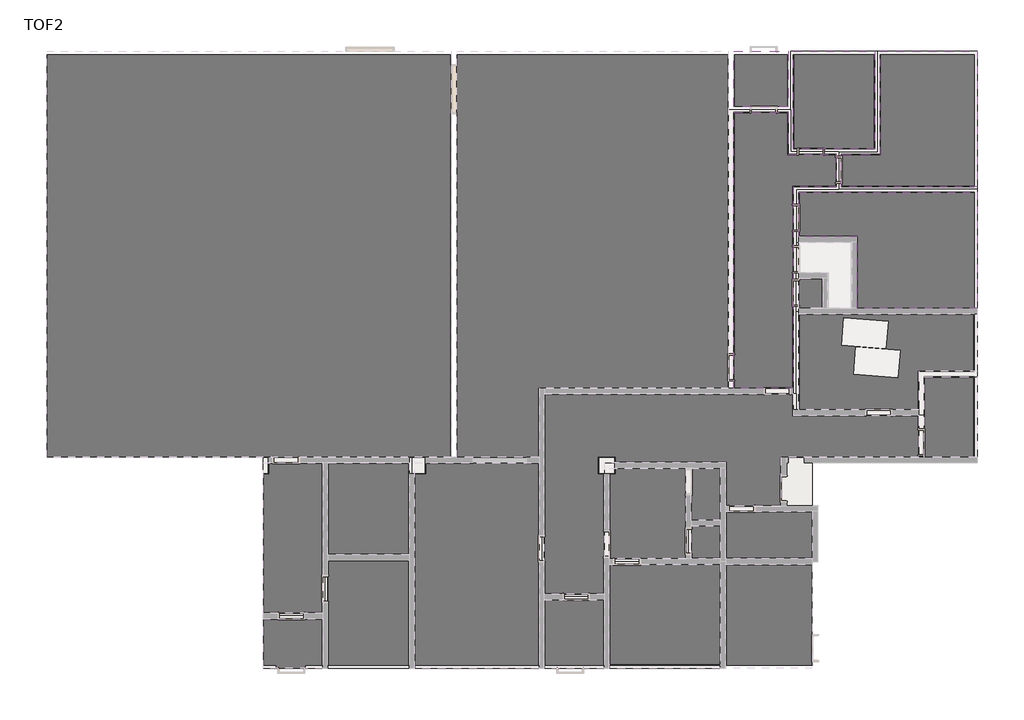
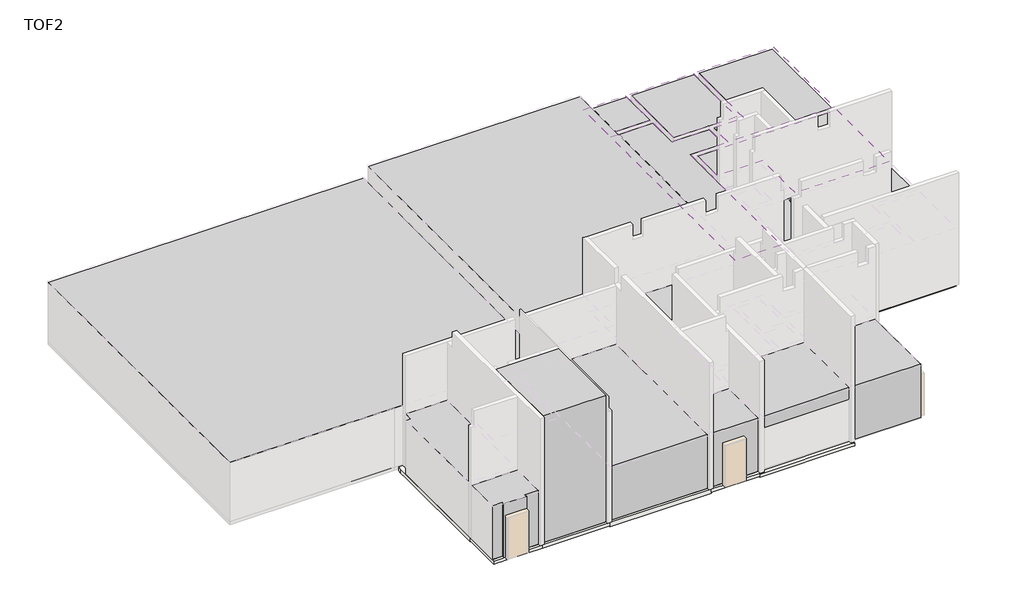
# One storey, part 5 of 5: 24 slabs, 23 proxies, 5 coverings.
# Revit data of these elements (continued)
# Room at (9390, 17931.521) mm, phase "New Construction", upper level "TOC", upper offset 2000 mm, lower offset -1000 mm (continued)
#   H_Ceiling-Base Material-5 = ""
#   H_Ceiling Finish-1 = "Acrylic Emulsion Paint"
#   H_Ceiling Finish-2 = ""
#   H_Ceiling Finish Remark = "SACE"
#   H_Room W = 17700 mm
#   H_Room L = 11400 mm
#   H_Room H or CH = 7300 mm
#   Floor Finish Style No = F06A
#   Skirt Finish Style No = B03
#   Wall Finish Style No = W01B
#   Ceiling Finish Style No = C01
# Room at (9390, 6347.521) mm, phase "New Construction", upper level "TOC", upper offset 2000 mm, lower offset -1000 mm
#   Comments = ""
#   Number = "112"
#   Name = "ELECTRICAL ROOM(SS08)"
#   H_Floor Finish Style Name = "Non-Slip Epoxy Paint"
#   H_Floor Base Material = "Concrete Slab / Screed"
#   H_Wall-Base Material-1 = "Masonry Wall"
#   H_Skirt Finish Style Name = "Epoxy Paint"
#   H_Wall-Base Material-2 = ""
#   H_Wall-Base Material-3 = "Plastering"
#   H_Floor-Base Material-1 = "Concrete Slab"
#   H_Floor-Base Material-2 = ""
#   H_Floor-Base Material-3 = "Screed"
#   H_Floor-Base Material-4 = ""
#   H_Floor-Base Material-5 = ""
#   H_Floor Finish-1 = "Epoxy Paint"
#   H_Floor Finish-2 = ""
#   H_Floor Finish Remark = "*WM 기준 확인 필요 Epoxy Paint \n(용제형, 0.1mm 이하) : epoxy resin + polyamine hardener(경화제)"
#   H_Skirt Base Material = "Same as Wall"
#   H_Skirt-Base Material-1 = ""
#   H_Skirt-Base Material-2 = ""
#   H_Skirt-Base Material-3 = ""
#   H_Skirt-Base Material-4 = ""
#   H_Skirt-Base Material-5 = ""
#   H_Skirt Finish-1 = "Epoxy Paint"
#   H_Skirt Finish-2 = ""
#   H_Skirt Finish Remark = "SACE"
#   H_Wall Finish Style Name = "Acrylic Emulsion Paint"
#   H_Wall Base Material = "Masonry Wall / Cement Plaster"
#   H_Wall-Base Material-4 = ""
#   H_Wall-Base Material-5 = ""
#   H_Wall Finish-1 = "Acrylic Emulsion Paint"
#   H_Wall Finish-2 = ""
#   H_Wall Finish Remark = "T13 Plaster"
#   H_Ceiling Finish Style Name = "Acrylic Emulsion Paint"
#   H_Ceiling Base Material = "Concrete Slab / Fair Faced Concrete"
#   H_Ceiling-Base Material-1 = "(Concrete Slab)"
#   H_Ceiling-Base Material-2 = ""
#   H_Ceiling-Base Material-3 = ""
#   H_Ceiling-Base Material-4 = ""
#   H_Ceiling-Base Material-5 = ""
#   H_Ceiling Finish-1 = "Acrylic Emulsion Paint"
#   H_Ceiling Finish-2 = ""
#   H_Ceiling Finish Remark = "SACE"
#   H_Room W = 17700 mm
#   H_Room L = 11000 mm
#   H_Room H or CH = 7300 mm
#   Floor Finish Style No = F06B
#   Skirt Finish Style No = B03
#   Wall Finish Style No = W01B
#   Ceiling Finish Style No = C01
# Room at (25850, 15981.521) mm, phase "New Construction", upper level "TOC", upper offset 2000 mm, lower offset 0 mm
#   Comments = ""
#   Number = "102"
#   Name = "RACK ROOM"
#   H_Floor Finish Style Name = "Anti-Dust Epoxy Paint / Anti-Static Vinyl Tile on Raised Floor"
#   H_Floor Base Material = "Concrete Slab / Steel Trowel Finish"
#   H_Wall-Base Material-1 = "Masonry Wall"
#   H_Skirt Finish Style Name = "Coved Vinyl Tile"
#   H_Wall-Base Material-2 = ""
#   H_Wall-Base Material-3 = "Plastering"
#   H_Floor-Base Material-1 = "Concrete Slab"
#   H_Floor-Base Material-2 = "Steel Trowel Finish"
#   H_Floor-Base Material-3 = ""
#   H_Floor-Base Material-4 = ""
#   H_Floor-Base Material-5 = "Raised Floor_Anti-Static Vinyl Tile"
#   H_Floor Finish-1 = "Anti-Dust Paint"
#   H_Floor Finish-2 = "Raised Floor_Anti-Static Vinyl Tile"
#   H_Floor Finish Remark = "600x600, H=1000"
#   H_Skirt Base Material = "Same as Wall"
#   H_Skirt-Base Material-1 = ""
#   H_Skirt-Base Material-2 = ""
#   H_Skirt-Base Material-3 = ""
#   H_Skirt-Base Material-4 = ""
#   H_Skirt-Base Material-5 = ""
#   H_Skirt Finish-1 = "Vinyl Tile"
#   H_Skirt Finish-2 = ""
#   H_Skirt Finish Remark = "Vinyl Tile = PVC Tile (polyvinyl chloride)"
#   H_Wall Finish Style Name = "Acrylic Emulsion Paint"
#   H_Wall Base Material = "Masonry Wall / Cement Plaster"
#   H_Wall-Base Material-4 = ""
#   H_Wall-Base Material-5 = ""
#   H_Wall Finish-1 = "Acrylic Emulsion Paint"
#   H_Wall Finish-2 = ""
#   H_Wall Finish Remark = "T13 Plaster"
#   H_Ceiling Finish Style Name = "Suspended Acoustic Tiled Ceiling (M-Bar)"
#   H_Ceiling Base Material = "Concrete Slab / Fair Faced Concrete"
#   H_Ceiling-Base Material-1 = "(Concrete Slab)"
#   H_Ceiling-Base Material-2 = "(Fair Faced Concrete)"
#   H_Ceiling-Base Material-3 = ""
#   H_Ceiling-Base Material-4 = ""
#   H_Ceiling-Base Material-5 = "Acoustic Tiled Ceiling System (M-Bar)"
#   H_Ceiling Finish-1 = "Acoustic Tiled Ceiling System (M-Bar)"
#   H_Ceiling Finish-2 = ""
#   H_Ceiling Finish Remark = ""
#   H_Room W = 14900 mm
#   H_Room L = 14900 mm
#   H_Room H or CH = 3000 mm
#   Floor Finish Style No = F91
#   Skirt Finish Style No = B35
#   Wall Finish Style No = W01B
#   Ceiling Finish Style No = C95A
# Room at (22100, 4784.521) mm, phase "New Construction", upper level "TOC", upper offset 2000 mm, lower offset -1000 mm
#   Comments = ""
#   Number = "114"
#   Name = "BATTERY ROOM"
#   H_Floor Finish Style Name = "Acid Resistant Ceramic Tile"
#   H_Floor Base Material = "Concrete Slab / Steel Trowel Finish"
#   H_Wall-Base Material-1 = "Masonry Wall"
#   H_Skirt Finish Style Name = "Coved Vinyl Tile"
#   H_Wall-Base Material-2 = ""
#   H_Wall-Base Material-3 = "Plastering"
#   H_Floor-Base Material-1 = "Concrete Slab"
#   H_Floor-Base Material-2 = "Steel Trowel Finish"
#   H_Floor-Base Material-3 = ""
#   H_Floor-Base Material-4 = ""
#   H_Floor-Base Material-5 = "Acid/Alkaline Resistant Tile"
#   H_Floor Finish-1 = "Acid/Alkaline Resistant Tile"
#   H_Floor Finish-2 = ""
#   H_Floor Finish Remark = "*WM : Bonding용 Mortar은 Tile에 포함\n*Slope 용 Screed만 별도 구분 (Concrete 바닥 단차 발생하는 경우 Only)"
#   H_Skirt Base Material = "Same as Wall"
#   H_Skirt-Base Material-1 = ""
#   H_Skirt-Base Material-2 = ""
#   H_Skirt-Base Material-3 = ""
#   H_Skirt-Base Material-4 = ""
#   H_Skirt-Base Material-5 = ""
#   H_Skirt Finish-1 = "Vinyl Tile"
#   H_Skirt Finish-2 = ""
#   H_Skirt Finish Remark = "Vinyl Tile = PVC Tile (polyvinyl chloride)"
#   H_Wall Finish Style Name = "Acid Resistant Paint"
#   H_Wall Base Material = "Masonry Wall / Cement Plaster"
#   H_Wall-Base Material-4 = ""
#   H_Wall-Base Material-5 = ""
#   H_Wall Finish-1 = "Acid/Alkaline Resistant Paint"
#   H_Wall Finish-2 = ""
#   H_Wall Finish Remark = "T13 Plaster"
#   H_Ceiling Finish Style Name = "Acrylic Emulsion Paint"
#   H_Ceiling Base Material = "Concrete Slab / Fair Faced Concrete"
#   H_Ceiling-Base Material-1 = "(Concrete Slab)"
#   H_Ceiling-Base Material-2 = ""
#   H_Ceiling-Base Material-3 = ""
#   H_Ceiling-Base Material-4 = ""
#   H_Ceiling-Base Material-5 = ""
#   H_Ceiling Finish-1 = "Acrylic Emulsion Paint"
#   H_Ceiling Finish-2 = ""
#   H_Ceiling Finish Remark = "SACE"
#   H_Room W = 7700 mm
#   H_Room L = 7500 mm
#   H_Room H or CH = 7300 mm
#   Floor Finish Style No = F32A
#   Skirt Finish Style No = B35
#   Wall Finish Style No = W04B
#   Ceiling Finish Style No = C01
# Room at (34305, 4784.521) mm, phase "New Construction", upper level "TOC", upper offset 2000 mm, lower offset 0 mm
#   Comments = ""
#   Number = "118"
#   Name = "DRIVERS LOUNGE"
#   H_Floor Finish Style Name = "Vinyl Tile"
#   H_Floor Base Material = "Concrete Slab / Steel Trowel Finish"
#   H_Wall-Base Material-1 = "Masonry Wall"
#   H_Skirt Finish Style Name = "Coved Vinyl Tile"
#   H_Wall-Base Material-2 = ""
#   H_Wall-Base Material-3 = "Plastering"
#   H_Floor-Base Material-1 = "Concrete Slab"
#   H_Floor-Base Material-2 = "Steel Trowel Finish"
#   H_Floor-Base Material-3 = ""
#   H_Floor-Base Material-4 = ""
#   H_Floor-Base Material-5 = "Vinyl Tile"
#   H_Floor Finish-1 = "Vinyl Tile"
#   H_Floor Finish-2 = ""
#   H_Floor Finish Remark = ""
#   H_Skirt Base Material = "Same as Wall"
#   H_Skirt-Base Material-1 = ""
#   H_Skirt-Base Material-2 = ""
#   H_Skirt-Base Material-3 = ""
#   H_Skirt-Base Material-4 = ""
#   H_Skirt-Base Material-5 = ""
#   H_Skirt Finish-1 = "Vinyl Tile"
#   H_Skirt Finish-2 = ""
#   H_Skirt Finish Remark = "Vinyl Tile = PVC Tile (polyvinyl chloride)"
#   H_Wall Finish Style Name = "Acrylic Emulsion Paint"
#   H_Wall Base Material = "Masonry Wall / Cement Plaster"
#   H_Wall-Base Material-4 = ""
#   H_Wall-Base Material-5 = ""
#   H_Wall Finish-1 = "Acrylic Emulsion Paint"
#   H_Wall Finish-2 = ""
#   H_Wall Finish Remark = "T13 Plaster"
#   H_Ceiling Finish Style Name = "Suspended Acoustic Tiled Ceiling (M-Bar)"
#   H_Ceiling Base Material = "Concrete Slab / Fair Faced Concrete"
#   H_Ceiling-Base Material-1 = "(Concrete Slab)"
#   H_Ceiling-Base Material-2 = "(Fair Faced Concrete)"
#   H_Ceiling-Base Material-3 = ""
#   H_Ceiling-Base Material-4 = ""
#   H_Ceiling-Base Material-5 = "Acoustic Tiled Ceiling System (M-Bar)"
#   H_Ceiling Finish-1 = "Acoustic Tiled Ceiling System (M-Bar)"
#   H_Ceiling Finish-2 = ""
#   H_Ceiling Finish Remark = ""
#   H_Room W = 4500 mm
#   H_Room L = 7500 mm
#   H_Room H or CH = 2600 mm
#   Floor Finish Style No = F34A
#   Skirt Finish Style No = B35
#   Wall Finish Style No = W01B
#   Ceiling Finish Style No = C95A
# Room at (38540.953, 16104.521) mm, phase "New Construction", upper level "TOC", upper offset 2000 mm, lower offset 0 mm
#   Comments = ""
#   Number = "103"
#   Name = "CONTROL ROOM"
#   H_Floor Finish Style Name = "Anti-Dust Epoxy Paint / Anti-Static Vinyl Tile on Raised Floor"
#   H_Floor Base Material = "Concrete Slab / Steel Trowel Finish"
#   H_Wall-Base Material-1 = "Masonry Wall"
#   H_Skirt Finish Style Name = "Coved Vinyl Tile"
#   H_Wall-Base Material-2 = ""
#   H_Wall-Base Material-3 = "Plastering"
#   H_Floor-Base Material-1 = "Concrete Slab"
#   H_Floor-Base Material-2 = "Steel Trowel Finish"
#   H_Floor-Base Material-3 = ""
#   H_Floor-Base Material-4 = ""
#   H_Floor-Base Material-5 = "Raised Floor_Anti-Static Vinyl Tile"
#   H_Floor Finish-1 = "Anti-Dust Paint"
#   H_Floor Finish-2 = "Raised Floor_Anti-Static Vinyl Tile"
#   H_Floor Finish Remark = "600x600, H=1000"
#   H_Skirt Base Material = "Same as Wall"
#   H_Skirt-Base Material-1 = ""
#   H_Skirt-Base Material-2 = ""
#   H_Skirt-Base Material-3 = ""
#   H_Skirt-Base Material-4 = ""
#   H_Skirt-Base Material-5 = ""
#   H_Skirt Finish-1 = "Vinyl Tile"
#   H_Skirt Finish-2 = ""
#   H_Skirt Finish Remark = "Vinyl Tile = PVC Tile (polyvinyl chloride)"
#   H_Wall Finish Style Name = "Acrylic Emulsion Paint"
#   H_Wall Base Material = "Masonry Wall / Cement Plaster"
#   H_Wall-Base Material-4 = ""
#   H_Wall-Base Material-5 = ""
#   H_Wall Finish-1 = "Acrylic Emulsion Paint"
#   H_Wall Finish-2 = ""
#   H_Wall Finish Remark = "T13 Plaster"
#   H_Ceiling Finish Style Name = "Suspended Acoustic Tiled Ceiling (M-Bar)"
#   H_Ceiling Base Material = "Concrete Slab / Fair Faced Concrete"
#   H_Ceiling-Base Material-1 = "(Concrete Slab)"
#   H_Ceiling-Base Material-2 = "(Fair Faced Concrete)"
#   H_Ceiling-Base Material-3 = ""
#   H_Ceiling-Base Material-4 = ""
#   H_Ceiling-Base Material-5 = "Acoustic Tiled Ceiling System (M-Bar)"
#   H_Ceiling Finish-1 = "Acoustic Tiled Ceiling System (M-Bar)"
#   H_Ceiling Finish-2 = ""
#   H_Ceiling Finish Remark = ""
#   H_Room W = 10000 mm
#   H_Room L = 14900 mm
#   H_Room H or CH = 3500 mm
#   Floor Finish Style No = F91
#   Skirt Finish Style No = B35
#   Wall Finish Style No = W01B
#   Ceiling Finish Style No = C95A
# Room at (41150, 2419.673) mm, phase "New Construction", upper level "TOC", upper offset 2000 mm, lower offset 0 mm
#   Comments = ""
#   Number = "122"
#   Name = "TOILETS"
#   H_Floor Finish Style Name = "Non-Slip Unglazed Ceramic Tile"
#   H_Floor Base Material = "Concrete Slab / Screed / Liquid Waterproofing"
#   H_Wall-Base Material-1 = "Masonry Wall"
#   H_Skirt Finish Style Name = "Coved Ceramic Tile"
#   H_Wall-Base Material-2 = ""
#   H_Wall-Base Material-3 = ""
#   H_Floor-Base Material-1 = "Concrete Slab"
#   H_Floor-Base Material-2 = ""
#   H_Floor-Base Material-3 = "Screed"
#   H_Floor-Base Material-4 = "Liquid Waterproofing"
#   H_Floor-Base Material-5 = "Ceramic Tile"
#   H_Floor Finish-1 = "Ceramic Tile"
#   H_Floor Finish-2 = ""
#   H_Floor Finish Remark = ""
#   H_Skirt Base Material = "Same as Wall"
#   H_Skirt-Base Material-1 = ""
#   H_Skirt-Base Material-2 = ""
#   H_Skirt-Base Material-3 = ""
#   H_Skirt-Base Material-4 = ""
#   H_Skirt-Base Material-5 = ""
#   H_Skirt Finish-1 = "Glazed Ceramic Tile"
#   H_Skirt Finish-2 = ""
#   H_Skirt Finish Remark = ""
#   H_Wall Finish Style Name = "Glazed Ceramic Tile (≤C.H+100) / No Paint (>C.H+100)"
#   H_Wall Base Material = "Masonry Wall / Liquid Waterproofing"
#   H_Wall-Base Material-4 = "Liquid Waterproofing"
#   H_Wall-Base Material-5 = "Glazed Ceramic Tile"
#   H_Wall Finish-1 = "Glazed Ceramic Tile"
#   H_Wall Finish-2 = ""
#   H_Wall Finish Remark = "Below Suspended Ceiling\nGlazed Ceramic Tile(≤C.H+100) + Liquid Waterproofing / No Paint (>C.H+100)"
#   H_Ceiling Finish Style Name = "Suspended Moisture Resistant Tiled Ceiling (M-Bar)"
#   H_Ceiling Base Material = "Concrete Slab / Fair Faced Concrete"
#   H_Ceiling-Base Material-1 = "(Concrete Slab)"
#   H_Ceiling-Base Material-2 = "(Fair Faced Concrete)"
#   H_Ceiling-Base Material-3 = ""
#   H_Ceiling-Base Material-4 = ""
#   H_Ceiling-Base Material-5 = "Moisture Resistant Tiled Ceiling System (M-Bar)"
#   H_Ceiling Finish-1 = "Moisture Resistant Tiled Ceiling System (M-Bar)"
#   H_Ceiling Finish-2 = ""
#   H_Ceiling Finish Remark = ""
#   H_Room W = 4000 mm
#   H_Room L = 3700 mm
#   H_Room H or CH = 2600 mm
#   Floor Finish Style No = F31B
#   Skirt Finish Style No = B32
#   Wall Finish Style No = W32B
#   Ceiling Finish Style No = C96A
# Room at (49742.5, 4429.521) mm, phase "New Construction", upper level "TOC", upper offset 2000 mm, lower offset -1000 mm
#   Comments = ""
#   Number = "125"
#   Name = "MAINTENANCE WORKSHOP"
#   H_Floor Finish Style Name = "Non-Slip Epoxy Paint"
#   H_Floor Base Material = "Concrete Slab / Steel Trowel Finish"
#   H_Wall-Base Material-1 = "Masonry Wall"
#   H_Skirt Finish Style Name = "Epoxy Paint"
#   H_Wall-Base Material-2 = ""
#   H_Wall-Base Material-3 = "Plastering"
#   H_Floor-Base Material-1 = "Concrete Slab"
#   H_Floor-Base Material-2 = "Steel Trowel Finish"
#   H_Floor-Base Material-3 = ""
#   H_Floor-Base Material-4 = ""
#   H_Floor-Base Material-5 = ""
#   H_Floor Finish-1 = "Epoxy Paint"
#   H_Floor Finish-2 = ""
#   H_Floor Finish Remark = "*WM 기준 확인 필요 Epoxy Paint \n(용제형, 0.1mm 이하) : epoxy resin + polyamine hardener(경화제)"
#   H_Skirt Base Material = "Same as Wall"
#   H_Skirt-Base Material-1 = ""
#   H_Skirt-Base Material-2 = ""
#   H_Skirt-Base Material-3 = ""
#   H_Skirt-Base Material-4 = ""
#   H_Skirt-Base Material-5 = ""
#   H_Skirt Finish-1 = "Epoxy Paint"
#   H_Skirt Finish-2 = ""
#   H_Skirt Finish Remark = "SACE"
#   H_Wall Finish Style Name = "Acrylic Emulsion Paint"
#   H_Wall Base Material = "Masonry Wall / Cement Plaster"
#   H_Wall-Base Material-4 = ""
#   H_Wall-Base Material-5 = ""
#   H_Wall Finish-1 = "Acrylic Emulsion Paint"
#   H_Wall Finish-2 = ""
#   H_Wall Finish Remark = "T13 Plaster"
#   H_Ceiling Finish Style Name = "Acrylic Emulsion Paint"
#   H_Ceiling Base Material = "Concrete Slab / Fair Faced Concrete"
#   H_Ceiling-Base Material-1 = "(Concrete Slab)"
#   H_Ceiling-Base Material-2 = ""
#   H_Ceiling-Base Material-3 = ""
#   H_Ceiling-Base Material-4 = ""
#   H_Ceiling-Base Material-5 = ""
#   H_Ceiling Finish-1 = "Acrylic Emulsion Paint"
#   H_Ceiling Finish-2 = ""
#   H_Ceiling Finish Remark = "SACE"
#   H_Room W = 6900 mm
#   H_Room L = 7500 mm
#   H_Room H or CH = 7300 mm
#   Floor Finish Style No = F06A
#   Skirt Finish Style No = B03
#   Wall Finish Style No = W01B
#   Ceiling Finish Style No = C01
# Room at (40470, 6702.369) mm, phase "New Construction", upper level "TOC", upper offset 2000 mm, lower offset 0 mm
#   Comments = ""
#   Number = "121"
#   Name = "LOCKER"
#   H_Floor Finish Style Name = "Non-Slip Unglazed Ceramic Tile"
#   H_Floor Base Material = "Concrete Slab / Steel Trowel Finish"
#   H_Wall-Base Material-1 = "Masonry Wall"
#   H_Skirt Finish Style Name = "Coved Ceramic Tile"
#   H_Wall-Base Material-2 = ""
#   H_Wall-Base Material-3 = ""
#   H_Floor-Base Material-1 = "Concrete Slab"
#   H_Floor-Base Material-2 = "Steel Trowel Finish"
#   H_Floor-Base Material-3 = ""
#   H_Floor-Base Material-4 = ""
#   H_Floor-Base Material-5 = "Ceramic Tile"
#   H_Floor Finish-1 = "Ceramic Tile"
#   H_Floor Finish-2 = ""
#   H_Floor Finish Remark = "*WM : Bonding용 Mortar은 Tile에 포함\n*Slope 용 Screed만 별도 구분 (Concrete 바닥 단차 발생하는 경우 Only)"
#   H_Skirt Base Material = "Same as Wall"
#   H_Skirt-Base Material-1 = ""
#   H_Skirt-Base Material-2 = ""
#   H_Skirt-Base Material-3 = ""
#   H_Skirt-Base Material-4 = ""
#   H_Skirt-Base Material-5 = ""
#   H_Skirt Finish-1 = "Glazed Ceramic Tile"
#   H_Skirt Finish-2 = ""
#   H_Skirt Finish Remark = ""
#   H_Wall Finish Style Name = "Glazed Ceramic Tile (≤C.H+100) / No Paint (>C.H+100)"
#   H_Wall Base Material = "Masonry Wall / Liquid Waterproofing"
#   H_Wall-Base Material-4 = "Liquid Waterproofing"
#   H_Wall-Base Material-5 = "Glazed Ceramic Tile"
#   H_Wall Finish-1 = "Glazed Ceramic Tile"
#   H_Wall Finish-2 = ""
#   H_Wall Finish Remark = "Below Suspended Ceiling\nGlazed Ceramic Tile(≤C.H+100) + Liquid Waterproofing / No Paint (>C.H+100)"
#   H_Ceiling Finish Style Name = "Suspended Moisture Resistant Tiled Ceiling (M-Bar)"
#   H_Ceiling Base Material = "Concrete Slab / Fair Faced Concrete"
#   H_Ceiling-Base Material-1 = "(Concrete Slab)"
#   H_Ceiling-Base Material-2 = "(Fair Faced Concrete)"
#   H_Ceiling-Base Material-3 = ""
#   H_Ceiling-Base Material-4 = ""
#   H_Ceiling-Base Material-5 = "Moisture Resistant Tiled Ceiling System (M-Bar)"
#   H_Ceiling Finish-1 = "Moisture Resistant Tiled Ceiling System (M-Bar)"
#   H_Ceiling Finish-2 = ""
#   H_Ceiling Finish Remark = ""
#   H_Room W = 2800 mm
#   H_Room L = 3300 mm
#   H_Room H or CH = 2700 mm
#   Floor Finish Style No = F31A
#   Skirt Finish Style No = B32
#   Wall Finish Style No = W32B
#   Ceiling Finish Style No = C96A
# Room at (42630, 7074.521) mm, phase "New Construction", upper level "TOC", upper offset 2000 mm, lower offset 0 mm
#   Comments = ""
#   Number = "127"
#   Name = "SHOWER ROOM"
#   H_Floor Finish Style Name = "Non-Slip Unglazed Ceramic Tile"
#   H_Floor Base Material = "Concrete Slab / Screed / Liquid Waterproofing"
#   H_Wall-Base Material-1 = "Concrete Wall"
#   H_Skirt Finish Style Name = "Epoxy Paint"
#   H_Wall-Base Material-2 = ""
#   H_Wall-Base Material-3 = ""
#   H_Floor-Base Material-1 = "Concrete Slab"
#   H_Floor-Base Material-2 = ""
#   H_Floor-Base Material-3 = "Screed"
#   H_Floor-Base Material-4 = "Liquid Waterproofing"
#   H_Floor-Base Material-5 = "Ceramic Tile"
#   H_Floor Finish-1 = "Ceramic Tile"
#   H_Floor Finish-2 = ""
#   H_Floor Finish Remark = ""
#   H_Skirt Base Material = "Same as Wall"
#   H_Skirt-Base Material-1 = ""
#   H_Skirt-Base Material-2 = ""
#   H_Skirt-Base Material-3 = ""
#   H_Skirt-Base Material-4 = ""
#   H_Skirt-Base Material-5 = ""
#   H_Skirt Finish-1 = "Epoxy Paint"
#   H_Skirt Finish-2 = ""
#   H_Skirt Finish Remark = "SACE"
#   H_Wall Finish Style Name = "Glazed Ceramic Tile (≤C.H+100) / No Paint (>C.H+100)"
#   H_Wall Base Material = "Concrete Wall"
#   H_Wall-Base Material-4 = "No Waterproofing"
#   H_Wall-Base Material-5 = "Glazed Ceramic Tile"
#   H_Wall Finish-1 = "Glazed Ceramic Tile"
#   H_Wall Finish-2 = ""
#   H_Wall Finish Remark = "Below Suspended Ceiling\nGlazed Ceramic Tile(≤C.H+100) / No Paint (>C.H+100)"
#   H_Ceiling Finish Style Name = "Suspended Moisture Resistant Tiled Ceiling (M-Bar)"
#   H_Ceiling Base Material = "Concrete Slab / Fair Faced Concrete"
#   H_Ceiling-Base Material-1 = "(Concrete Slab)"
#   H_Ceiling-Base Material-2 = "(Fair Faced Concrete)"
#   H_Ceiling-Base Material-3 = ""
#   H_Ceiling-Base Material-4 = ""
#   H_Ceiling-Base Material-5 = "Moisture Resistant Tiled Ceiling System (M-Bar)"
#   H_Ceiling Finish-1 = "Moisture Resistant Tiled Ceiling System (M-Bar)"
#   H_Ceiling Finish-2 = ""
#   H_Ceiling Finish Remark = ""
#   H_Room W = 1000 mm
#   H_Room L = 1900 mm
#   H_Room H or CH = 2600 mm
#   Floor Finish Style No = F31B
#   Skirt Finish Style No = B03
#   Wall Finish Style No = W32C
#   Ceiling Finish Style No = C96A
# Room at (42695, 5872.369) mm, phase "New Construction", upper level "TOC", upper offset 2000 mm, lower offset 0 mm
#   Comments = ""
#   Number = "128"
#   Name = "EWH ROOM"
#   H_Floor Finish Style Name = "Non-Slip Unglazed Ceramic Tile"
#   H_Floor Base Material = "Concrete Slab / Steel Trowel Finish"
#   H_Wall-Base Material-1 = "Masonry Wall"
#   H_Skirt Finish Style Name = "Epoxy Paint"
#   H_Wall-Base Material-2 = ""
#   H_Wall-Base Material-3 = "Plastering"
#   H_Floor-Base Material-1 = "Concrete Slab"
#   H_Floor-Base Material-2 = "Steel Trowel Finish"
#   H_Floor-Base Material-3 = ""
#   H_Floor-Base Material-4 = ""
#   H_Floor-Base Material-5 = "Ceramic Tile"
#   H_Floor Finish-1 = "Ceramic Tile"
#   H_Floor Finish-2 = ""
#   H_Floor Finish Remark = "*WM : Bonding용 Mortar은 Tile에 포함\n*Slope 용 Screed만 별도 구분 (Concrete 바닥 단차 발생하는 경우 Only)"
#   H_Skirt Base Material = "Same as Wall"
#   H_Skirt-Base Material-1 = ""
#   H_Skirt-Base Material-2 = ""
#   H_Skirt-Base Material-3 = ""
#   H_Skirt-Base Material-4 = ""
#   H_Skirt-Base Material-5 = ""
#   H_Skirt Finish-1 = "Epoxy Paint"
#   H_Skirt Finish-2 = ""
#   H_Skirt Finish Remark = "SACE"
#   H_Wall Finish Style Name = "Acrylic Emulsion Paint"
#   H_Wall Base Material = "Masonry Wall / Cement Plaster"
#   H_Wall-Base Material-4 = ""
#   H_Wall-Base Material-5 = ""
#   H_Wall Finish-1 = "Acrylic Emulsion Paint"
#   H_Wall Finish-2 = ""
#   H_Wall Finish Remark = "T13 Plaster"
#   H_Ceiling Finish Style Name = "Suspended Acoustic Tiled Ceiling (M-Bar)"
#   H_Ceiling Base Material = "Concrete Slab / Fair Faced Concrete"
#   H_Ceiling-Base Material-1 = "(Concrete Slab)"
#   H_Ceiling-Base Material-2 = "(Fair Faced Concrete)"
#   H_Ceiling-Base Material-3 = ""
#   H_Ceiling-Base Material-4 = ""
#   H_Ceiling-Base Material-5 = "Acoustic Tiled Ceiling System (M-Bar)"
#   H_Ceiling Finish-1 = "Acoustic Tiled Ceiling System (M-Bar)"
#   H_Ceiling Finish-2 = ""
#   H_Ceiling Finish Remark = ""
#   H_Room W = 1000 mm
#   H_Room L = 1200 mm
#   H_Room H or CH = 2700 mm
#   Floor Finish Style No = F31A
#   Skirt Finish Style No = B03
#   Wall Finish Style No = W01B
#   Ceiling Finish Style No = C95A
# Room at (52032, 10149.521) mm, phase "New Construction", upper level "TOC", upper offset 2000 mm, lower offset 0 mm
#   Comments = ""
#   Number = "110"
#   Name = "ABLUTIONS"
#   H_Floor Finish Style Name = "Non-Slip Unglazed Ceramic Tile"
#   H_Floor Base Material = "Concrete Slab / Screed / Liquid Waterproofing"
#   H_Wall-Base Material-1 = "Masonry Wall"
#   H_Skirt Finish Style Name = "Coved Ceramic Tile"
#   H_Wall-Base Material-2 = ""
#   H_Wall-Base Material-3 = ""
#   H_Floor-Base Material-1 = "Concrete Slab"
#   H_Floor-Base Material-2 = ""
#   H_Floor-Base Material-3 = "Screed"
#   H_Floor-Base Material-4 = "Liquid Waterproofing"
#   H_Floor-Base Material-5 = "Ceramic Tile"
#   H_Floor Finish-1 = "Ceramic Tile"
#   H_Floor Finish-2 = ""
#   H_Floor Finish Remark = ""
#   H_Skirt Base Material = "Same as Wall"
#   H_Skirt-Base Material-1 = ""
#   H_Skirt-Base Material-2 = ""
#   H_Skirt-Base Material-3 = ""
#   H_Skirt-Base Material-4 = ""
#   H_Skirt-Base Material-5 = ""
#   H_Skirt Finish-1 = "Glazed Ceramic Tile"
#   H_Skirt Finish-2 = ""
#   H_Skirt Finish Remark = ""
#   H_Wall Finish Style Name = "Glazed Ceramic Tile (≤C.H+100) / No Paint (>C.H+100)"
#   H_Wall Base Material = "Masonry Wall / Liquid Waterproofing"
#   H_Wall-Base Material-4 = "Liquid Waterproofing"
#   H_Wall-Base Material-5 = "Glazed Ceramic Tile"
#   H_Wall Finish-1 = "Glazed Ceramic Tile"
#   H_Wall Finish-2 = ""
#   H_Wall Finish Remark = "Below Suspended Ceiling\nGlazed Ceramic Tile(≤C.H+100) + Liquid Waterproofing / No Paint (>C.H+100)"
#   H_Ceiling Finish Style Name = "Suspended Moisture Resistant Tiled Ceiling (M-Bar)"
#   H_Ceiling Base Material = "Concrete Slab / Fair Faced Concrete"
#   H_Ceiling-Base Material-1 = "(Concrete Slab)"
#   H_Ceiling-Base Material-2 = "(Fair Faced Concrete)"
#   H_Ceiling-Base Material-3 = ""
#   H_Ceiling-Base Material-4 = ""
#   H_Ceiling-Base Material-5 = "Moisture Resistant Tiled Ceiling System (M-Bar)"
#   H_Ceiling Finish-1 = "Moisture Resistant Tiled Ceiling System (M-Bar)"
#   H_Ceiling Finish-2 = ""
#   H_Ceiling Finish Remark = ""
#   H_Room W = 1800 mm
#   H_Room L = 2900 mm
#   H_Room H or CH = 2600 mm
#   Floor Finish Style No = F31B
#   Skirt Finish Style No = B32
#   Wall Finish Style No = W32B
#   Ceiling Finish Style No = C96A
# Room at (50280, 21414.521) mm, phase "New Construction", upper level "TOC", upper offset 2000 mm, lower offset 0 mm
#   Comments = ""
#   Number = "106"
#   Name = "SHIFT SUPERVISOR/DAY SUPERVISOR"
#   H_Floor Finish Style Name = "Vinyl Tile"
#   H_Floor Base Material = "Concrete Slab / Steel Trowel Finish"
#   H_Wall-Base Material-1 = "Masonry Wall"
#   H_Skirt Finish Style Name = "Coved Vinyl Tile"
#   H_Wall-Base Material-2 = ""
#   H_Wall-Base Material-3 = "Plastering"
#   H_Floor-Base Material-1 = "Concrete Slab"
#   H_Floor-Base Material-2 = "Steel Trowel Finish"
#   H_Floor-Base Material-3 = ""
#   H_Floor-Base Material-4 = ""
#   H_Floor-Base Material-5 = "Vinyl Tile"
#   H_Floor Finish-1 = "Vinyl Tile"
#   H_Floor Finish-2 = ""
#   H_Floor Finish Remark = ""
#   H_Skirt Base Material = "Same as Wall"
#   H_Skirt-Base Material-1 = ""
#   H_Skirt-Base Material-2 = ""
#   H_Skirt-Base Material-3 = ""
#   H_Skirt-Base Material-4 = ""
#   H_Skirt-Base Material-5 = ""
#   H_Skirt Finish-1 = "Vinyl Tile"
#   H_Skirt Finish-2 = ""
#   H_Skirt Finish Remark = "Vinyl Tile = PVC Tile (polyvinyl chloride)"
#   H_Wall Finish Style Name = "Acrylic Emulsion Paint"
#   H_Wall Base Material = "Masonry Wall / Cement Plaster"
#   H_Wall-Base Material-4 = ""
#   H_Wall-Base Material-5 = ""
#   H_Wall Finish-1 = "Acrylic Emulsion Paint"
#   H_Wall Finish-2 = ""
#   H_Wall Finish Remark = "T13 Plaster"
#   H_Ceiling Finish Style Name = "Suspended Acoustic Tiled Ceiling (M-Bar)"
#   H_Ceiling Base Material = "Concrete Slab / Fair Faced Concrete"
#   H_Ceiling-Base Material-1 = "(Concrete Slab)"
#   H_Ceiling-Base Material-2 = "(Fair Faced Concrete)"
#   H_Ceiling-Base Material-3 = ""
#   H_Ceiling-Base Material-4 = ""
#   H_Ceiling-Base Material-5 = "Acoustic Tiled Ceiling System (M-Bar)"
#   H_Ceiling Finish-1 = "Acoustic Tiled Ceiling System (M-Bar)"
#   H_Ceiling Finish-2 = ""
#   H_Ceiling Finish Remark = ""
#   H_Room W = 4900 mm
#   H_Room L = 4900 mm
#   H_Room H or CH = 2600 mm
#   Floor Finish Style No = F34A
#   Skirt Finish Style No = B35
#   Wall Finish Style No = W01B
#   Ceiling Finish Style No = C95A
# Room at (44795, 22494.021) mm, phase "New Construction", upper level "TOC", upper offset 2000 mm, lower offset 0 mm
#   Comments = ""
#   Number = "104"
#   Name = "AIR LOCK"
#   H_Floor Finish Style Name = "Vinyl Tile"
#   H_Floor Base Material = "Concrete Slab / Steel Trowel Finish"
#   H_Wall-Base Material-1 = "Masonry Wall"
#   H_Skirt Finish Style Name = "Coved Vinyl Tile"
#   H_Wall-Base Material-2 = ""
#   H_Wall-Base Material-3 = "Plastering"
#   H_Floor-Base Material-1 = "Concrete Slab"
#   H_Floor-Base Material-2 = "Steel Trowel Finish"
#   H_Floor-Base Material-3 = ""
#   H_Floor-Base Material-4 = ""
#   H_Floor-Base Material-5 = "Vinyl Tile"
#   H_Floor Finish-1 = "Vinyl Tile"
#   H_Floor Finish-2 = ""
#   H_Floor Finish Remark = ""
#   H_Skirt Base Material = "Same as Wall"
#   H_Skirt-Base Material-1 = ""
#   H_Skirt-Base Material-2 = ""
#   H_Skirt-Base Material-3 = ""
#   H_Skirt-Base Material-4 = ""
#   H_Skirt-Base Material-5 = ""
#   H_Skirt Finish-1 = "Vinyl Tile"
#   H_Skirt Finish-2 = ""
#   H_Skirt Finish Remark = "Vinyl Tile = PVC Tile (polyvinyl chloride)"
#   H_Wall Finish Style Name = "Acrylic Emulsion Paint"
#   H_Wall Base Material = "Masonry Wall / Cement Plaster"
#   H_Wall-Base Material-4 = ""
#   H_Wall-Base Material-5 = ""
#   H_Wall Finish-1 = "Acrylic Emulsion Paint"
#   H_Wall Finish-2 = ""
#   H_Wall Finish Remark = "T13 Plaster"
#   H_Ceiling Finish Style Name = "Suspended Acoustic Tiled Ceiling (M-Bar)"
#   H_Ceiling Base Material = "Concrete Slab / Fair Faced Concrete"
#   H_Ceiling-Base Material-1 = "(Concrete Slab)"
#   H_Ceiling-Base Material-2 = "(Fair Faced Concrete)"
#   H_Ceiling-Base Material-3 = ""
#   H_Ceiling-Base Material-4 = ""
#   H_Ceiling-Base Material-5 = "Acoustic Tiled Ceiling System (M-Bar)"
#   H_Ceiling Finish-1 = "Acoustic Tiled Ceiling System (M-Bar)"
#   H_Ceiling Finish-2 = ""
#   H_Ceiling Finish Remark = ""
#   H_Room W = 1900 mm
#   H_Room L = 1900 mm
#   H_Room H or CH = 2600 mm
#   Floor Finish Style No = F34A
#   Skirt Finish Style No = B35
#   Wall Finish Style No = W01B
#   Ceiling Finish Style No = C95A
# Room at (45465, 16437.021) mm, phase "New Construction", upper level "TOC", upper offset 2000 mm, lower offset 0 mm
#   Comments = ""
#   Number = "107"
#   Name = "CORRIDOR"
#   H_Floor Finish Style Name = "Vinyl Tile"
#   H_Floor Base Material = "Concrete Slab / Steel Trowel Finish"
#   H_Wall-Base Material-1 = "Masonry Wall"
#   H_Skirt Finish Style Name = "Coved Vinyl Tile"
#   H_Wall-Base Material-2 = ""
#   H_Wall-Base Material-3 = "Plastering"
#   H_Floor-Base Material-1 = "Concrete Slab"
#   H_Floor-Base Material-2 = "Steel Trowel Finish"
#   H_Floor-Base Material-3 = ""
#   H_Floor-Base Material-4 = ""
#   H_Floor-Base Material-5 = "Vinyl Tile"
#   H_Floor Finish-1 = "Vinyl Tile"
#   H_Floor Finish-2 = ""
#   H_Floor Finish Remark = ""
#   H_Skirt Base Material = "Same as Wall"
#   H_Skirt-Base Material-1 = ""
#   H_Skirt-Base Material-2 = ""
#   H_Skirt-Base Material-3 = ""
#   H_Skirt-Base Material-4 = ""
#   H_Skirt-Base Material-5 = ""
#   H_Skirt Finish-1 = "Vinyl Tile"
#   H_Skirt Finish-2 = ""
#   H_Skirt Finish Remark = "Vinyl Tile = PVC Tile (polyvinyl chloride)"
#   H_Wall Finish Style Name = "Acrylic Emulsion Paint"
#   H_Wall Base Material = "Masonry Wall / Cement Plaster"
#   H_Wall-Base Material-4 = ""
#   H_Wall-Base Material-5 = ""
#   H_Wall Finish-1 = "Acrylic Emulsion Paint"
#   H_Wall Finish-2 = ""
#   H_Wall Finish Remark = "T13 Plaster"
#   H_Ceiling Finish Style Name = "Suspended Acoustic Tiled Ceiling (M-Bar)"
#   H_Ceiling Base Material = "Concrete Slab / Fair Faced Concrete"
#   H_Ceiling-Base Material-1 = "(Concrete Slab)"
#   H_Ceiling-Base Material-2 = "(Fair Faced Concrete)"
#   H_Ceiling-Base Material-3 = ""
#   H_Ceiling-Base Material-4 = ""
#   H_Ceiling-Base Material-5 = "Acoustic Tiled Ceiling System (M-Bar)"
#   H_Ceiling Finish-1 = "Acoustic Tiled Ceiling System (M-Bar)"
#   H_Ceiling Finish-2 = ""
#   H_Ceiling Finish Remark = ""
#   H_Room W = 3700 mm
#   H_Room L = 10100 mm
#   H_Room H or CH = 2600 mm
#   Floor Finish Style No = F34A
#   Skirt Finish Style No = B35
#   Wall Finish Style No = W01B
#   Ceiling Finish Style No = C95A
# Room at (47300, 21676.521) mm, phase "New Construction", upper level "TOC", upper offset 2000 mm, lower offset 0 mm
#   Comments = ""
#   Number = "105"
#   Name = "LIBRARY"
#   H_Floor Finish Style Name = "Vinyl Tile"
#   H_Floor Base Material = "Concrete Slab / Steel Trowel Finish"
#   H_Wall-Base Material-1 = "Masonry Wall"
#   H_Skirt Finish Style Name = "Coved Vinyl Tile"
#   H_Wall-Base Material-2 = ""
#   H_Wall-Base Material-3 = "Plastering"
#   H_Floor-Base Material-1 = "Concrete Slab"
#   H_Floor-Base Material-2 = "Steel Trowel Finish"
#   H_Floor-Base Material-3 = ""
#   H_Floor-Base Material-4 = ""
#   H_Floor-Base Material-5 = "Vinyl Tile"
#   H_Floor Finish-1 = "Vinyl Tile"
#   H_Floor Finish-2 = ""
#   H_Floor Finish Remark = ""
#   H_Skirt Base Material = "Same as Wall"
#   H_Skirt-Base Material-1 = ""
#   H_Skirt-Base Material-2 = ""
#   H_Skirt-Base Material-3 = ""
#   H_Skirt-Base Material-4 = ""
#   H_Skirt-Base Material-5 = ""
#   H_Skirt Finish-1 = "Vinyl Tile"
#   H_Skirt Finish-2 = ""
#   H_Skirt Finish Remark = "Vinyl Tile = PVC Tile (polyvinyl chloride)"
#   H_Wall Finish Style Name = "Acrylic Emulsion Paint"
#   H_Wall Base Material = "Masonry Wall / Cement Plaster"
#   H_Wall-Base Material-4 = ""
#   H_Wall-Base Material-5 = ""
#   H_Wall Finish-1 = "Acrylic Emulsion Paint"
#   H_Wall Finish-2 = ""
#   H_Wall Finish Remark = "T13 Plaster"
#   H_Ceiling Finish Style Name = "Suspended Acoustic Tiled Ceiling (M-Bar)"
#   H_Ceiling Base Material = "Concrete Slab / Fair Faced Concrete"
#   H_Ceiling-Base Material-1 = "(Concrete Slab)"
#   H_Ceiling-Base Material-2 = "(Fair Faced Concrete)"
#   H_Ceiling-Base Material-3 = ""
#   H_Ceiling-Base Material-4 = ""
#   H_Ceiling-Base Material-5 = "Acoustic Tiled Ceiling System (M-Bar)"
#   H_Ceiling Finish-1 = "Acoustic Tiled Ceiling System (M-Bar)"
#   H_Ceiling Finish-2 = ""
#   H_Ceiling Finish Remark = ""
#   H_Room W = 2900 mm
#   H_Room L = 3500 mm
#   H_Room H or CH = 2600 mm
#   Floor Finish Style No = F34A
#   Skirt Finish Style No = B35
#   Wall Finish Style No = W01B
#   Ceiling Finish Style No = C95A
# Room at (49372, 12124.521) mm, phase "New Construction", upper level "TOC", upper offset 2000 mm, lower offset 0 mm
#   Comments = ""
#   Number = "111"
#   Name = "PRAYER ROOM"
#   H_Floor Finish Style Name = "Carpet Tile"
#   H_Floor Base Material = "Concrete Slab / Steel Trowel Finish"
#   H_Wall-Base Material-1 = "Masonry Wall"
#   H_Skirt Finish Style Name = "Coved Vinyl Tile"
#   H_Wall-Base Material-2 = ""
#   H_Wall-Base Material-3 = "Plastering"
#   H_Floor-Base Material-1 = "Concrete Slab"
#   H_Floor-Base Material-2 = ""
#   H_Floor-Base Material-3 = "Screed"
#   H_Floor-Base Material-5 = "Carpet Tile"
#   H_Floor Finish-1 = "Carpet Tile"
#   H_Skirt Base Material = "Same as Wall"
#   H_Skirt-Base Material-1 = ""
#   H_Skirt-Base Material-2 = ""
#   H_Skirt-Base Material-3 = ""
#   H_Skirt-Base Material-4 = ""
#   H_Skirt-Base Material-5 = ""
#   H_Skirt Finish-1 = "Vinyl Tile"
#   H_Skirt Finish-2 = ""
#   H_Skirt Finish Remark = "Vinyl Tile = PVC Tile (polyvinyl chloride)"
#   H_Wall Finish Style Name = "Acrylic Emulsion Paint"
#   H_Wall Base Material = "Masonry Wall / Cement Plaster"
#   H_Wall-Base Material-4 = ""
#   H_Wall-Base Material-5 = ""
#   H_Wall Finish-1 = "Acrylic Emulsion Paint"
#   H_Wall Finish-2 = ""
#   H_Wall Finish Remark = "T13 Plaster"
#   H_Ceiling Finish Style Name = "Suspended Acoustic Tiled Ceiling (M-Bar)"
#   H_Ceiling Base Material = "Concrete Slab / Fair Faced Concrete"
#   H_Ceiling-Base Material-1 = "(Concrete Slab)"
#   H_Ceiling-Base Material-2 = "(Fair Faced Concrete)"
#   H_Ceiling-Base Material-3 = ""
#   H_Ceiling-Base Material-4 = ""
#   H_Ceiling-Base Material-5 = "Acoustic Tiled Ceiling System (M-Bar)"
#   H_Ceiling Finish-1 = "Acoustic Tiled Ceiling System (M-Bar)"
#   H_Ceiling Finish-2 = ""
#   H_Ceiling Finish Remark = ""
#   H_Room W = 6400 mm
#   H_Room L = 3500 mm
#   H_Room H or CH = 2600 mm
#   Floor Finish Style No = F43-1
#   Skirt Finish Style No = B35
#   Wall Finish Style No = W01B
#   Ceiling Finish Style No = C95A
# Room at (49620, 16249.521) mm, phase "New Construction", upper level "TOC", upper offset 2000 mm, lower offset 0 mm
#   Comments = ""
#   Number = "108"
#   Name = "BREAK ROOM"
#   H_Floor Finish Style Name = "Vinyl Tile"
#   H_Floor Base Material = "Concrete Slab / Steel Trowel Finish"
#   H_Wall-Base Material-1 = "Masonry Wall"
#   H_Skirt Finish Style Name = "Coved Vinyl Tile"
#   H_Wall-Base Material-2 = ""
#   H_Wall-Base Material-3 = "Plastering"
#   H_Floor-Base Material-1 = "Concrete Slab"
#   H_Floor-Base Material-2 = "Steel Trowel Finish"
#   H_Floor-Base Material-3 = ""
#   H_Floor-Base Material-4 = ""
#   H_Floor-Base Material-5 = "Vinyl Tile"
#   H_Floor Finish-1 = "Vinyl Tile"
#   H_Floor Finish-2 = ""
#   H_Floor Finish Remark = ""
#   H_Skirt Base Material = "Same as Wall"
#   H_Skirt-Base Material-1 = ""
#   H_Skirt-Base Material-2 = ""
#   H_Skirt-Base Material-3 = ""
#   H_Skirt-Base Material-4 = ""
#   H_Skirt-Base Material-5 = ""
#   H_Skirt Finish-1 = "Vinyl Tile"
#   H_Skirt Finish-2 = ""
#   H_Skirt Finish Remark = "Vinyl Tile = PVC Tile (polyvinyl chloride)"
#   H_Wall Finish Style Name = "Acrylic Emulsion Paint"
#   H_Wall Base Material = "Masonry Wall / Cement Plaster"
#   H_Wall-Base Material-4 = ""
#   H_Wall-Base Material-5 = ""
#   H_Wall Finish-1 = "Acrylic Emulsion Paint"
#   H_Wall Finish-2 = ""
#   H_Wall Finish Remark = "T13 Plaster"
#   H_Ceiling Finish Style Name = "Suspended Moisture Resistant Tiled Ceiling (M-Bar)"
#   H_Ceiling Base Material = "Concrete Slab / Fair Faced Concrete"
#   H_Ceiling-Base Material-1 = "(Concrete Slab)"
#   H_Ceiling-Base Material-2 = "(Fair Faced Concrete)"
#   H_Ceiling-Base Material-3 = ""
#   H_Ceiling-Base Material-4 = ""
#   H_Ceiling-Base Material-5 = "Moisture Resistant Tiled Ceiling System (M-Bar)"
#   H_Ceiling Finish-1 = "Moisture Resistant Tiled Ceiling System (M-Bar)"
#   H_Ceiling Finish-2 = ""
#   H_Ceiling Finish Remark = ""
#   H_Room W = 6500 mm
#   H_Room L = 4200 mm
#   H_Room H or CH = 2600 mm
#   Floor Finish Style No = F34A
#   Skirt Finish Style No = B35
#   Wall Finish Style No = W01B
#   Ceiling Finish Style No = C96A
# Room at (47333.247, 15516.296) mm, phase "New Construction", upper level "TOC", upper offset 2000 mm, lower offset 0 mm
#   Comments = ""
#   Number = "109"
#   Name = "JANITOR"
#   H_Floor Finish Style Name = "Non-Slip Unglazed Ceramic Tile"
#   H_Floor Base Material = "Concrete Slab / Screed / Liquid Waterproofing"
#   H_Wall-Base Material-1 = "Masonry Wall"
#   H_Skirt Finish Style Name = "Coved Ceramic Tile"
#   H_Wall-Base Material-2 = ""
#   H_Wall-Base Material-3 = ""
#   H_Floor-Base Material-1 = "Concrete Slab"
#   H_Floor-Base Material-2 = ""
#   H_Floor-Base Material-3 = "Screed"
#   H_Floor-Base Material-4 = "Liquid Waterproofing"
#   H_Floor-Base Material-5 = "Ceramic Tile"
#   H_Floor Finish-1 = "Ceramic Tile"
#   H_Floor Finish-2 = ""
#   H_Floor Finish Remark = ""
#   H_Skirt Base Material = "Same as Wall"
#   H_Skirt-Base Material-1 = ""
#   H_Skirt-Base Material-2 = ""
#   H_Skirt-Base Material-3 = ""
#   H_Skirt-Base Material-4 = ""
#   H_Skirt-Base Material-5 = ""
#   H_Skirt Finish-1 = "Glazed Ceramic Tile"
#   H_Skirt Finish-2 = ""
#   H_Skirt Finish Remark = ""
#   H_Wall Finish Style Name = "Glazed Ceramic Tile (≤C.H+100) / No Paint (>C.H+100)"
#   H_Wall Base Material = "Masonry Wall / Liquid Waterproofing"
#   H_Wall-Base Material-4 = "Liquid Waterproofing"
#   H_Wall-Base Material-5 = "Glazed Ceramic Tile"
#   H_Wall Finish-1 = "Glazed Ceramic Tile"
#   H_Wall Finish-2 = ""
#   H_Wall Finish Remark = "Below Suspended Ceiling\nGlazed Ceramic Tile(≤C.H+100) + Liquid Waterproofing / No Paint (>C.H+100)"
#   H_Ceiling Finish Style Name = "Suspended Moisture Resistant Tiled Ceiling (M-Bar)"
#   H_Ceiling Base Material = "Concrete Slab / Fair Faced Concrete"
#   H_Ceiling-Base Material-1 = "(Concrete Slab)"
#   H_Ceiling-Base Material-2 = "(Fair Faced Concrete)"
#   H_Ceiling-Base Material-3 = ""
#   H_Ceiling-Base Material-4 = ""
#   H_Ceiling-Base Material-5 = "Moisture Resistant Tiled Ceiling System (M-Bar)"
#   H_Ceiling Finish-1 = "Moisture Resistant Tiled Ceiling System (M-Bar)"
#   H_Ceiling Finish-2 = ""
#   H_Ceiling Finish Remark = ""
#   H_Room W = 800 mm
#   H_Room L = 1100 mm
#   H_Room H or CH = 2600 mm
#   Floor Finish Style No = F31B
#   Skirt Finish Style No = B32
#   Wall Finish Style No = W32B
#   Ceiling Finish Style No = C96A
# Room at (46580, 14657.021) mm, phase "New Construction", upper level "TOC", upper offset 2000 mm, lower offset 0 mm
#   Comments = ""
#   Number = "126"
#   Name = "EWH ROOM"
#   H_Floor Finish Style Name = "Vinyl Tile"
#   H_Floor Base Material = "Concrete Slab / Steel Trowel Finish"
#   H_Wall-Base Material-1 = "Masonry Wall"
#   H_Skirt Finish Style Name = "Coved Vinyl Tile"
#   H_Wall-Base Material-2 = ""
#   H_Wall-Base Material-3 = "Plastering"
#   H_Floor-Base Material-1 = "Concrete Slab"
#   H_Floor-Base Material-2 = "Steel Trowel Finish"
#   H_Floor-Base Material-3 = ""
#   H_Floor-Base Material-4 = ""
#   H_Floor-Base Material-5 = "Vinyl Tile"
#   H_Floor Finish-1 = "Vinyl Tile"
#   H_Floor Finish-2 = ""
#   H_Floor Finish Remark = ""
#   H_Skirt Base Material = "Same as Wall"
#   H_Skirt-Base Material-1 = ""
#   H_Skirt-Base Material-2 = ""
#   H_Skirt-Base Material-3 = ""
#   H_Skirt-Base Material-4 = ""
#   H_Skirt-Base Material-5 = ""
#   H_Skirt Finish-1 = "Vinyl Tile"
#   H_Skirt Finish-2 = ""
#   H_Skirt Finish Remark = "Vinyl Tile = PVC Tile (polyvinyl chloride)"
#   H_Wall Finish Style Name = "Acrylic Emulsion Paint"
#   H_Wall Base Material = "Masonry Wall / Cement Plaster"
#   H_Wall-Base Material-4 = ""
#   H_Wall-Base Material-5 = ""
#   H_Wall Finish-1 = "Acrylic Emulsion Paint"
#   H_Wall Finish-2 = ""
#   H_Wall Finish Remark = "T13 Plaster"
#   H_Ceiling Finish Style Name = "Suspended Acoustic Tiled Ceiling (M-Bar)"
#   H_Ceiling Base Material = "Concrete Slab / Fair Faced Concrete"
#   H_Ceiling-Base Material-1 = "(Concrete Slab)"
#   H_Ceiling-Base Material-2 = "(Fair Faced Concrete)"
#   H_Ceiling-Base Material-3 = ""
#   H_Ceiling-Base Material-4 = ""
#   H_Ceiling-Base Material-5 = "Acoustic Tiled Ceiling System (M-Bar)"
#   H_Ceiling Finish-1 = "Acoustic Tiled Ceiling System (M-Bar)"
#   H_Ceiling Finish-2 = ""
#   H_Ceiling Finish Remark = ""
#   H_Room W = 3100 mm
#   H_Room L = 1700 mm
#   H_Room H or CH = 2600 mm
#   Floor Finish Style No = F34A
#   Skirt Finish Style No = B35
#   Wall Finish Style No = W01B
#   Ceiling Finish Style No = C95A
# Room at (45350, 5729.521) mm, phase "New Construction", upper level "TOC", upper offset 2000 mm, lower offset 0 mm
#   Comments = ""
#   Number = "123"
#   Name = "STORE"
#   H_Floor Finish Style Name = "Vinyl Tile"
#   H_Floor Base Material = "Concrete Slab / Steel Trowel Finish"
#   H_Wall-Base Material-1 = "Masonry Wall"
#   H_Skirt Finish Style Name = "Coved Vinyl Tile"
#   H_Wall-Base Material-2 = ""
#   H_Wall-Base Material-3 = "Plastering"
#   H_Floor-Base Material-1 = "Concrete Slab"
#   H_Floor-Base Material-2 = "Steel Trowel Finish"
#   H_Floor-Base Material-3 = ""
#   H_Floor-Base Material-4 = ""
#   H_Floor-Base Material-5 = "Vinyl Tile"
#   H_Floor Finish-1 = "Vinyl Tile"
#   H_Floor Finish-2 = ""
#   H_Floor Finish Remark = ""
#   H_Skirt Base Material = "Same as Wall"
#   H_Skirt-Base Material-1 = ""
#   H_Skirt-Base Material-2 = ""
#   H_Skirt-Base Material-3 = ""
#   H_Skirt-Base Material-4 = ""
#   H_Skirt-Base Material-5 = ""
#   H_Skirt Finish-1 = "Vinyl Tile"
#   H_Skirt Finish-2 = ""
#   H_Skirt Finish Remark = "Vinyl Tile = PVC Tile (polyvinyl chloride)"
#   H_Wall Finish Style Name = "Acrylic Emulsion Paint"
#   H_Wall Base Material = "Masonry Wall / Cement Plaster"
#   H_Wall-Base Material-4 = ""
#   H_Wall-Base Material-5 = ""
#   H_Wall Finish-1 = "Acrylic Emulsion Paint"
#   H_Wall Finish-2 = ""
#   H_Wall Finish Remark = "T13 Plaster"
#   H_Ceiling Finish Style Name = "Suspended Acoustic Tiled Ceiling (M-Bar)"
#   H_Ceiling Base Material = "Concrete Slab / Fair Faced Concrete"
#   H_Ceiling-Base Material-1 = "(Concrete Slab)"
#   H_Ceiling-Base Material-2 = "(Fair Faced Concrete)"
#   H_Ceiling-Base Material-3 = ""
#   H_Ceiling-Base Material-4 = ""
#   H_Ceiling-Base Material-5 = "Acoustic Tiled Ceiling System (M-Bar)"
#   H_Ceiling Finish-1 = "Acoustic Tiled Ceiling System (M-Bar)"
#   H_Ceiling Finish-2 = ""
#   H_Ceiling Finish Remark = ""
#   H_Room W = 3100 mm
#   H_Room L = 3700 mm
#   H_Room H or CH = 2600 mm
#   Floor Finish Style No = F34A
#   Skirt Finish Style No = B35
#   Wall Finish Style No = W01B
#   Ceiling Finish Style No = C95A
# Room at (45350, 2414.673) mm, phase "New Construction", upper level "TOC", upper offset 2000 mm, lower offset 0 mm
#   Comments = ""
#   Number = "124"
#   Name = "STORE"
#   H_Floor Finish Style Name = "Vinyl Tile"
#   H_Floor Base Material = "Concrete Slab / Steel Trowel Finish"
#   H_Wall-Base Material-1 = "Masonry Wall"
#   H_Skirt Finish Style Name = "Coved Vinyl Tile"
#   H_Wall-Base Material-2 = ""
#   H_Wall-Base Material-3 = "Plastering"
#   H_Floor-Base Material-1 = "Concrete Slab"
#   H_Floor-Base Material-2 = "Steel Trowel Finish"
#   H_Floor-Base Material-3 = ""
#   H_Floor-Base Material-4 = ""
#   H_Floor-Base Material-5 = "Vinyl Tile"
#   H_Floor Finish-1 = "Vinyl Tile"
#   H_Floor Finish-2 = ""
#   H_Floor Finish Remark = ""
#   H_Skirt Base Material = "Same as Wall"
#   H_Skirt-Base Material-1 = ""
#   H_Skirt-Base Material-2 = ""
#   H_Skirt-Base Material-3 = ""
#   H_Skirt-Base Material-4 = ""
#   H_Skirt-Base Material-5 = ""
#   H_Skirt Finish-1 = "Vinyl Tile"
#   H_Skirt Finish-2 = ""
#   H_Skirt Finish Remark = "Vinyl Tile = PVC Tile (polyvinyl chloride)"
#   H_Wall Finish Style Name = "Acrylic Emulsion Paint"
#   H_Wall Base Material = "Masonry Wall / Cement Plaster"
#   H_Wall-Base Material-4 = ""
#   H_Wall-Base Material-5 = ""
#   H_Wall Finish-1 = "Acrylic Emulsion Paint"
#   H_Wall Finish-2 = ""
#   H_Wall Finish Remark = "T13 Plaster"
#   H_Ceiling Finish Style Name = "Suspended Acoustic Tiled Ceiling (M-Bar)"
#   H_Ceiling Base Material = "Concrete Slab / Fair Faced Concrete"
#   H_Ceiling-Base Material-1 = "(Concrete Slab)"
#   H_Ceiling-Base Material-2 = "(Fair Faced Concrete)"
#   H_Ceiling-Base Material-3 = ""
#   H_Ceiling-Base Material-4 = ""
#   H_Ceiling-Base Material-5 = "Acoustic Tiled Ceiling System (M-Bar)"
#   H_Ceiling Finish-1 = "Acoustic Tiled Ceiling System (M-Bar)"
#   H_Ceiling Finish-2 = ""
#   H_Ceiling Finish Remark = ""
#   H_Room W = 2900 mm
#   H_Room L = 3900 mm
#   H_Room H or CH = 6300 mm
#   Floor Finish Style No = F34A
#   Skirt Finish Style No = B35
#   Wall Finish Style No = W01B
#   Ceiling Finish Style No = C95A
# Room at (30342.5, 2466.271) mm, phase "New Construction", upper level "TOC", upper offset 2000 mm, lower offset 0 mm
#   Comments = ""
#   Number = "115"
#   Name = "TELECOMS ROOM"
#   H_Floor Finish Style Name = "Vinyl Tile"
#   H_Floor Base Material = "Concrete Slab / Steel Trowel Finish"
#   H_Wall-Base Material-1 = "Masonry Wall"
#   H_Skirt Finish Style Name = "Coved Vinyl Tile"
#   H_Wall-Base Material-2 = ""
#   H_Wall-Base Material-3 = "Plastering"
#   H_Floor-Base Material-1 = "Concrete Slab"
#   H_Floor-Base Material-2 = "Steel Trowel Finish"
#   H_Floor-Base Material-3 = ""
#   H_Floor-Base Material-4 = ""
#   H_Floor-Base Material-5 = "Vinyl Tile"
#   H_Floor Finish-1 = "Vinyl Tile"
#   H_Floor Finish-2 = ""
#   H_Floor Finish Remark = ""
#   H_Skirt Base Material = "Same as Wall"
#   H_Skirt-Base Material-1 = ""
#   H_Skirt-Base Material-2 = ""
#   H_Skirt-Base Material-3 = ""
#   H_Skirt-Base Material-4 = ""
#   H_Skirt-Base Material-5 = ""
#   H_Skirt Finish-1 = "Vinyl Tile"
#   H_Skirt Finish-2 = ""
#   H_Skirt Finish Remark = "Vinyl Tile = PVC Tile (polyvinyl chloride)"
#   H_Wall Finish Style Name = "Latex Paint"
#   H_Wall Base Material = "Masonry Wall / Cement Plaster"
#   H_Wall-Base Material-4 = ""
#   H_Wall-Base Material-5 = ""
#   H_Wall Finish-1 = "Latex Paint"
#   H_Wall Finish-2 = ""
#   H_Wall Finish Remark = ""
#   H_Ceiling Finish Style Name = "Acrylic Emulsion Paint"
#   H_Ceiling Base Material = "Concrete Slab / Fair Faced Concrete"
#   H_Ceiling-Base Material-1 = "(Concrete Slab)"
#   H_Ceiling-Base Material-2 = ""
#   H_Ceiling-Base Material-3 = ""
#   H_Ceiling-Base Material-4 = ""
#   H_Ceiling-Base Material-5 = ""
#   H_Ceiling Finish-1 = "Acrylic Emulsion Paint"
#   H_Ceiling Finish-2 = ""
#   H_Ceiling Finish Remark = "SACE"
#   H_Room W = 2900 mm
#   H_Room L = 3300 mm
#   H_Room H or CH = 2600 mm
#   Floor Finish Style No = F34A
#   Skirt Finish Style No = B35
#   Wall Finish Style No = W03B
#   Ceiling Finish Style No = C01
# Room at (30057.5, 6598.271) mm, phase "New Construction", upper level "TOC", upper offset 2000 mm, lower offset 0 mm
#   Comments = ""
#   Number = "113"
#   Name = "STORE"
#   H_Floor Finish Style Name = "Vinyl Tile"
#   H_Floor Base Material = "Concrete Slab / Steel Trowel Finish"
#   H_Wall-Base Material-1 = "Masonry Wall"
#   H_Skirt Finish Style Name = "Coved Vinyl Tile"
#   H_Wall-Base Material-2 = ""
#   H_Wall-Base Material-3 = "Plastering"
#   H_Floor-Base Material-1 = "Concrete Slab"
#   H_Floor-Base Material-2 = "Steel Trowel Finish"
#   H_Floor-Base Material-3 = ""
#   H_Floor-Base Material-4 = ""
#   H_Floor-Base Material-5 = "Vinyl Tile"
#   H_Floor Finish-1 = "Vinyl Tile"
#   H_Floor Finish-2 = ""
#   H_Floor Finish Remark = ""
#   H_Skirt Base Material = "Same as Wall"
#   H_Skirt-Base Material-1 = ""
#   H_Skirt-Base Material-2 = ""
#   H_Skirt-Base Material-3 = ""
#   H_Skirt-Base Material-4 = ""
#   H_Skirt-Base Material-5 = ""
#   H_Skirt Finish-1 = "Vinyl Tile"
#   H_Skirt Finish-2 = ""
#   H_Skirt Finish Remark = "Vinyl Tile = PVC Tile (polyvinyl chloride)"
#   H_Wall Finish Style Name = "Acrylic Emulsion Paint"
#   H_Wall Base Material = "Masonry Wall / Cement Plaster"
#   H_Wall-Base Material-4 = ""
#   H_Wall-Base Material-5 = ""
#   H_Wall Finish-1 = "Acrylic Emulsion Paint"
#   H_Wall Finish-2 = ""
#   H_Wall Finish Remark = "T13 Plaster"
#   H_Ceiling Finish Style Name = "Suspended Acoustic Tiled Ceiling (M-Bar)"
#   H_Ceiling Base Material = "Concrete Slab / Fair Faced Concrete"
#   H_Ceiling-Base Material-1 = "(Concrete Slab)"
#   H_Ceiling-Base Material-2 = "(Fair Faced Concrete)"
#   H_Ceiling-Base Material-3 = ""
#   H_Ceiling-Base Material-4 = ""
#   H_Ceiling-Base Material-5 = "Acoustic Tiled Ceiling System (M-Bar)"
#   H_Ceiling Finish-1 = "Acoustic Tiled Ceiling System (M-Bar)"
#   H_Ceiling Finish-2 = ""
#   H_Ceiling Finish Remark = ""
#   H_Room W = 2100 mm
#   H_Room L = 1900 mm
#   H_Room H or CH = 2700 mm
